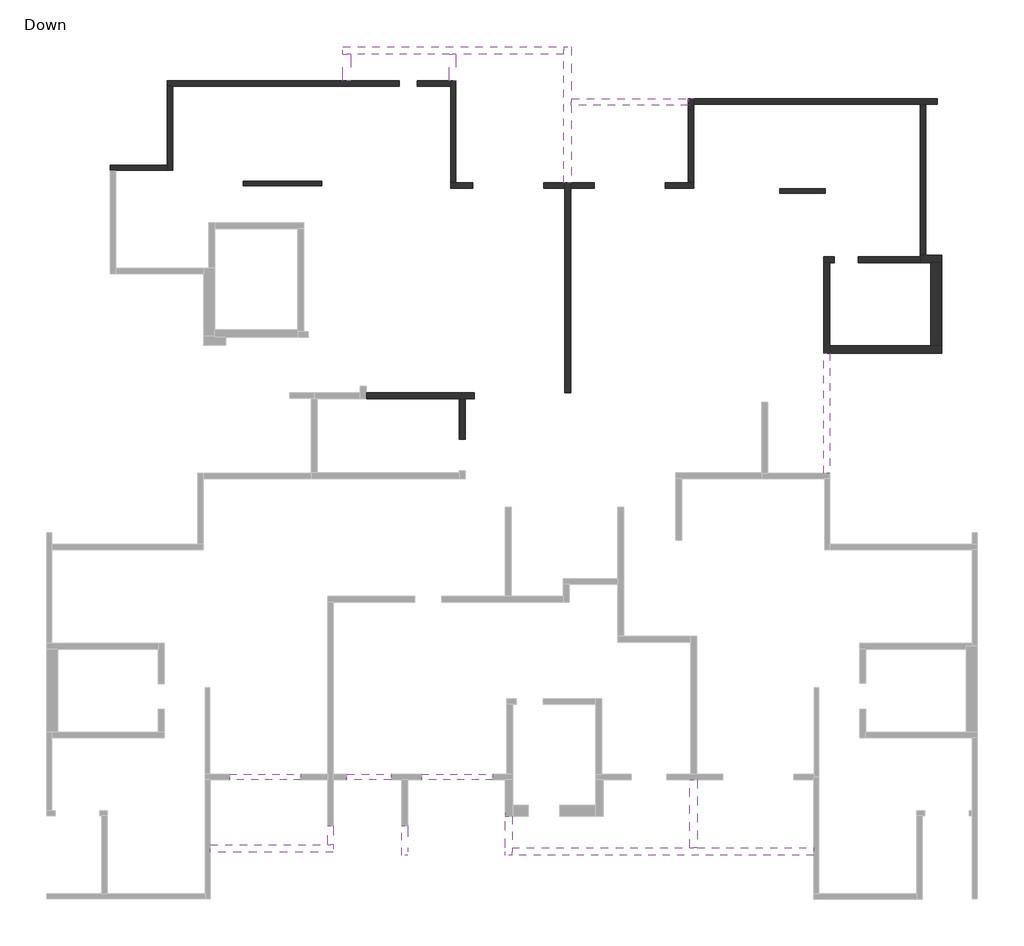
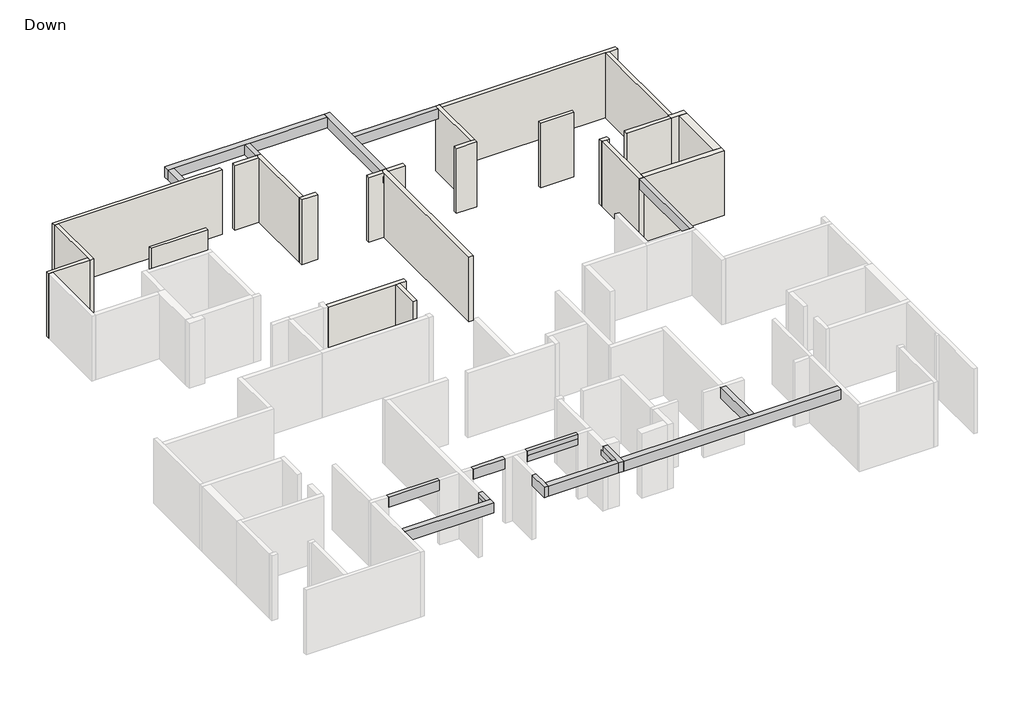
# One storey, part 3 of 3: 23 walls, 15 beams.
"""IFC4 building model written with IfcOpenShell, lengths in millimetres."""

from ifc_helpers import new_model, si_unit, frame, origin, place, context, project, spatial, polyline, outline, extrude, faceted_brep, element, save

model = new_model("IFC4")

# Units and contexts
model_context = context("Model", 3, world=origin())
ifc_project = project(units=[si_unit("LENGTHUNIT", "METRE", prefix="MILLI")], contexts=[model_context])

# Site, building, storey
site = spatial("IfcSite", under=ifc_project)
building = spatial("IfcBuilding", under=site)
storey = spatial("IfcBuildingStorey", under=building, Name="Down", Elevation=0.0)

# Beams
placement = place(None, origin())
element("IfcBeam", 1, ObjectType="Concrete Rectengular Beam : 18/50", at=placement, inside=storey, context=model_context, shape_type="Brep", body=[
    faceted_brep([(-10116.2830918, -11344.051338, 3200.0), (-10116.2830918, -11524.051338, 3200.0), (-10116.2830918, -11524.051338, 2700.0), (-10116.2830918, -11344.051338, 2700.0), (-10116.2830918, -11344.051338, 3000.0), (-12517.1627599, -11344.051338, 2700.0), (-12517.1627599, -11524.051338, 2700.0), (-12517.1627599, -11524.051338, 3200.0), (-12517.1627599, -11344.051338, 3200.0), (-12517.1627599, -11344.051338, 3000.0)], [[[0, 1, 2, 3, 4]], [[5, 6, 7, 8, 9]], [[1, 0, 8, 7]], [[2, 1, 7, 6]], [[3, 2, 6, 5]], [[8, 0, 4, 3, 5, 9]]]),
])
element("IfcBeam", 2, ObjectType="Concrete Rectengular Beam : 18/50", at=placement, inside=storey, context=model_context, shape_type="Brep", body=[
    faceted_brep([(-7066.175208, -11524.051338, 3200.0), (-7066.175208, -11344.051338, 3200.0), (-8566.988486, -11344.051338, 3200.0), (-8566.988486, -11524.051338, 3200.0), (-7066.175208, -11524.051338, 2700.0), (-8566.988486, -11524.051338, 2700.0), (-7066.175208, -11344.051338, 2700.0), (-8566.988486, -11344.051338, 2700.0), (-7066.175208, -11344.051338, 3000.0), (-8566.988486, -11344.051338, 3000.0)], [[[0, 1, 2, 3]], [[4, 0, 3, 5]], [[6, 4, 5, 7]], [[2, 1, 8, 6, 7, 9]], [[1, 0, 4, 6, 8]], [[3, 2, 9, 7, 5]]]),
])
element("IfcBeam", 3, ObjectType="Concrete Rectengular Beam : 18/50", at=placement, inside=storey, context=model_context, shape_type="Brep", body=[
    faceted_brep([(-3636.648237, -11344.051338, 3200.0), (-6035.4200213, -11344.051338, 3200.0), (-6035.4200213, -11519.051338, 3200.0), (-3636.648237, -11519.051338, 3200.0), (-6035.4200213, -11524.051338, 2700.0), (-3636.648237, -11524.051338, 2700.0), (-3636.648237, -11524.051338, 2980.0), (-6035.4200213, -11524.051338, 2980.0), (-3636.648237, -11344.051338, 2700.0), (-6035.4200213, -11344.051338, 2700.0), (-6035.4200213, -11344.051338, 3000.0), (-3636.648237, -11344.051338, 3000.0), (-3636.648237, -11519.051338, 2980.0), (-6035.4200213, -11519.051338, 2980.0)], [[[0, 1, 2, 3]], [[4, 5, 6, 7]], [[8, 5, 4, 9]], [[9, 10, 1, 0, 11, 8]], [[5, 8, 11, 0, 3, 12, 6]], [[9, 4, 7, 13, 2, 1, 10]], [[12, 13, 7, 6]], [[13, 12, 3, 2]]]),
])
element("IfcBeam", 4, ObjectType="Concrete Rectengular Beam : 20/50", at=placement, inside=storey, context=model_context, shape_type="SweptSolid", body=[
    extrude(outline(polyline([(2700.0, -9216.2167018), (2700.0, -9016.2167018), (3200.0, -9016.2167018), (3200.0, -9211.2167018), (2980.0, -9211.2167018), (2980.0, -9216.2167018), (2700.0, -9216.2167018)])), frame((0.0, -13713.3127488, 0.0), z_axis=(0.0, 1.0, 0.0), x_axis=(0.0, 0.0, 1.0)), (0.0, 0.0, 1.0), 645.0124481),
])
element("IfcBeam", 5, ObjectType="Concrete Rectengular Beam : 20/50", at=placement, inside=storey, context=model_context, shape_type="Brep", body=[
    faceted_brep([(-6516.0175316, -13068.3003006, 3200.0), (-6516.0175316, -13068.3003006, 2700.0), (-6716.0175316, -13068.3003006, 2700.0), (-6716.0175316, -13068.3003006, 3200.0), (-6716.0175316, -14074.491172, 3200.0), (-6516.0175316, -14074.491172, 3200.0), (-6516.0175316, -13814.491172, 3200.0), (-6716.0175316, -14074.491172, 2700.0), (-6516.0175316, -13814.491172, 2700.0), (-6516.0175316, -14074.491172, 2700.0)], [[[0, 1, 2, 3]], [[0, 3, 4, 5, 6]], [[3, 2, 7, 4]], [[2, 1, 8, 9, 7]], [[1, 0, 6, 5, 9, 8]], [[5, 4, 7, 9]]]),
])
element("IfcBeam", 6, ObjectType="Concrete Rectengular Beam : 20/50", at=placement, inside=storey, context=model_context, shape_type="Brep", body=[
    faceted_brep([(7535.1359953, -1184.051338, 3200.0), (7735.1359953, -1184.051338, 3200.0), (7735.1359953, 2875.7328944, 3200.0), (7535.1359953, 2875.7328944, 3200.0), (7535.1359953, -1184.051338, 2700.0), (7535.1359953, -1184.051338, 3000.0), (7535.1359953, 2875.7328944, 2700.0), (7735.1359953, -1184.051338, 2700.0), (7735.1359953, 2875.7328944, 2700.0)], [[[0, 1, 2, 3]], [[4, 5, 0, 3, 6]], [[7, 4, 6, 8]], [[1, 7, 8, 2]], [[1, 0, 5, 4, 7]], [[3, 2, 8, 6]]]),
])
element("IfcBeam", 7, ObjectType="Concrete Rectengular Beam : 22/50", at=placement, inside=storey, context=model_context, shape_type="Brep", body=[
    faceted_brep([(3133.8745845, 11456.9279151, 3200.0), (3133.8745845, 11457.7079981, 3200.0), (-986.7976146, 11457.7079981, 3200.0), (-986.7976146, 11237.7079981, 3200.0), (2953.8745845, 11237.7079981, 3200.0), (2953.8745845, 11456.9279151, 3200.0), (3133.8745845, 11457.7079981, 2700.0), (-986.7976146, 11457.7079981, 2700.0), (3133.8745845, 11456.9279151, 2700.0), (2953.8745845, 11456.9279151, 2700.0), (2953.8745845, 11237.7079981, 2700.0), (-986.7976146, 11237.7079981, 2700.0), (2953.8745845, 11237.7079981, 2980.0), (-986.7976146, 11237.7079981, 2980.0)], [[[0, 1, 2, 3, 4, 5]], [[1, 6, 7, 2]], [[6, 8, 9, 10, 11, 7]], [[10, 12, 4, 3, 13, 11]], [[6, 1, 0, 8]], [[9, 5, 4, 12, 10]], [[5, 9, 8, 0]], [[3, 2, 7, 11, 13]]]),
])
element("IfcBeam", 8, ObjectType="Concrete Rectengular Beam : 23/50", at=placement, inside=storey, context=model_context, shape_type="Brep", body=[
    faceted_brep([(-3216.3411831, -12636.8603469, 2700.0), (-3220.4458666, -12636.8603469, 2700.0), (-3220.4458666, -12636.8603469, 2980.0), (-3216.3411831, -12636.8603469, 2980.0), (-3220.4458666, -14074.491172, 3200.0), (-2990.4458666, -14074.491172, 3200.0), (-2990.4458666, -13814.491172, 3200.0), (-2990.4458666, -12754.2256118, 3200.0), (-3211.3411831, -12754.2256118, 3200.0), (-3211.3411831, -13814.491172, 3200.0), (-3220.4458666, -13814.491172, 3200.0), (-3220.4458666, -13814.491172, 2700.0), (-3220.4458666, -14074.491172, 2700.0), (-3220.4458666, -13814.491172, 2980.0), (-3216.3411831, -12754.2256118, 2700.0), (-2990.4458666, -12754.2256118, 2700.0), (-2990.4458666, -13814.491172, 2700.0), (-2990.4458666, -14074.491172, 2700.0), (-3216.3411831, -12754.2256118, 2980.0), (-3211.3411831, -12754.2256118, 2980.0), (-3211.3411831, -13814.491172, 2980.0)], [[[0, 1, 2, 3]], [[4, 5, 6, 7, 8, 9, 10]], [[1, 11, 12, 4, 10, 13, 2]], [[1, 0, 14, 15, 16, 17, 12, 11]], [[15, 7, 6, 5, 17, 16]], [[14, 0, 3, 18]], [[15, 14, 18, 19, 8, 7]], [[5, 4, 12, 17]], [[20, 19, 18, 3, 2, 13]], [[20, 9, 8, 19]], [[9, 20, 13, 10]]]),
])
element("IfcBeam", 9, ObjectType="Concrete Rectengular Beam : 23/50", at=placement, inside=storey, context=model_context, shape_type="Brep", body=[
    faceted_brep([(-5116.3826769, 12066.1063384, 3200.0), (-5065.7934653, 12066.1063384, 3200.0), (-4886.3826769, 12066.1063384, 3200.0), (-4886.3826769, 12957.7411932, 3200.0), (-5116.3826769, 12957.7411932, 3200.0), (-4886.3826769, 12957.7411932, 2700.0), (-4886.3826769, 12957.7411932, 2980.0), (-4886.3826769, 12066.1063384, 2980.0), (-4886.3826769, 12066.1063384, 2700.0), (-5116.3826769, 12066.1063384, 2700.0), (-5116.3826769, 12957.7411932, 2700.0), (-5116.3826769, 12066.1063384, 2980.0), (-5116.3826769, 12957.7411932, 2980.0)], [[[0, 1, 2, 3, 4]], [[5, 6, 3, 2, 7, 8]], [[8, 9, 10, 5]], [[9, 11, 0, 4, 12, 10]], [[0, 11, 9, 8, 7, 2, 1]], [[4, 3, 6, 5, 10, 12]]]),
])
element("IfcBeam", 10, ObjectType="Concrete Rectengular Beam : 26/50", at=placement, inside=storey, context=model_context, shape_type="Brep", body=[
    faceted_brep([(-13167.6689839, -13713.3127488, 3200.0), (-13167.6689839, -13973.3127488, 3200.0), (-9016.2167018, -13973.3127488, 3200.0), (-9016.2167018, -13713.3127488, 3200.0), (-9211.2167018, -13713.3127488, 3200.0), (-13167.6689839, -13973.3127488, 2700.0), (-9016.2167018, -13973.3127488, 2700.0), (-13167.6689839, -13713.3127488, 2700.0), (-9216.2167018, -13713.3127488, 2700.0), (-9016.2167018, -13713.3127488, 2700.0), (-13167.6689839, -13713.3127488, 2980.0)], [[[0, 1, 2, 3, 4]], [[1, 5, 6, 2]], [[5, 7, 8, 9, 6]], [[7, 10, 0, 4, 3, 9, 8]], [[1, 0, 10, 7, 5]], [[3, 2, 6, 9]]]),
])
element("IfcBeam", 11, ObjectType="Concrete Rectengular Beam : 26/50", at=placement, inside=storey, context=model_context, shape_type="Brep", body=[
    faceted_brep([(7185.3434642, -14074.491172, 3200.0), (7185.3434642, -13814.491172, 3200.0), (3265.0530078, -13814.491172, 3200.0), (3005.0530078, -13814.491172, 3200.0), (-2990.4458666, -13814.491172, 3200.0), (-2990.4458666, -14074.491172, 3200.0), (7185.3434642, -14074.491172, 2700.0), (-2990.4458666, -14074.491172, 2700.0), (7185.3434642, -13814.491172, 2700.0), (-2990.4458666, -13814.491172, 2700.0), (3005.0530078, -13814.491172, 2700.0), (3265.0530078, -13814.491172, 2700.0), (7185.3434642, -13814.491172, 2980.0)], [[[0, 1, 2, 3, 4, 5]], [[6, 0, 5, 7]], [[8, 6, 7, 9, 10, 11]], [[1, 12, 8, 11, 10, 9, 4, 3, 2]], [[1, 0, 6, 8, 12]], [[5, 4, 9, 7]]]),
    faceted_brep([(-6516.0175316, -14074.491172, 3200.0), (-6516.0175316, -13814.491172, 3200.0), (-6516.0175316, -13814.491172, 2980.0), (-6516.0175316, -13814.491172, 2700.0), (-6516.0175316, -14074.491172, 2700.0), (-3220.4458666, -13814.491172, 3200.0), (-3220.4458666, -14074.491172, 3200.0), (-3220.4458666, -14074.491172, 2700.0), (-3220.4458666, -13814.491172, 2700.0), (-3220.4458666, -13814.491172, 2980.0)], [[[0, 1, 2, 3, 4]], [[5, 6, 7, 8, 9]], [[1, 0, 6, 5]], [[0, 4, 7, 6]], [[4, 3, 8, 7]], [[3, 2, 1, 5, 9, 8]]]),
])
element("IfcBeam", 12, ObjectType="Concrete Rectengular Beam : 26/50", at=placement, inside=storey, context=model_context, shape_type="Brep", body=[
    faceted_brep([(3265.0530078, -11524.051338, 3200.0), (3005.0530078, -11524.051338, 3200.0), (3005.0530078, -13814.491172, 3200.0), (3265.0530078, -13814.491172, 3200.0), (3005.0530078, -11524.051338, 2700.0), (3005.0530078, -13814.491172, 2700.0), (3265.0530078, -11524.051338, 2700.0), (3265.0530078, -13814.491172, 2700.0), (3265.0530078, -11524.051338, 2980.0), (3265.0530078, -13814.491172, 2980.0)], [[[0, 1, 2, 3]], [[1, 4, 5, 2]], [[4, 6, 7, 5]], [[6, 8, 0, 3, 9, 7]], [[1, 0, 8, 6, 4]], [[3, 2, 5, 7, 9]]]),
])
element("IfcBeam", 13, ObjectType="Concrete Rectengular Beam : 26/50", at=placement, inside=storey, context=model_context, shape_type="Brep", body=[
    faceted_brep([(-1246.7976146, 8617.6084131, 3200.0), (-1216.7976146, 8617.6084131, 3200.0), (-1016.7976146, 8617.6084131, 3200.0), (-986.7976146, 8617.6084131, 3200.0), (-986.7976146, 11237.7079981, 3200.0), (-986.7976146, 11457.7079981, 3200.0), (-986.7976146, 13217.7411932, 3200.0), (-1246.7976146, 13217.7411932, 3200.0), (-1246.7976146, 12957.7411932, 3200.0), (-986.7976146, 8617.6084131, 2980.0), (-986.7976146, 8617.6084131, 2700.0), (-986.7976146, 11237.7079981, 2700.0), (-986.7976146, 11457.7079981, 2700.0), (-986.7976146, 13217.7411932, 2700.0), (-1246.7976146, 8617.6084131, 2700.0), (-1246.7976146, 12957.7411932, 2700.0), (-1246.7976146, 13217.7411932, 2700.0), (-1246.7976146, 8617.6084131, 2980.0)], [[[0, 1, 2, 3, 4, 5, 6, 7, 8]], [[3, 9, 10, 11, 12, 13, 6, 5, 4]], [[10, 14, 15, 16, 13, 12, 11]], [[0, 17, 14, 10, 9, 3, 2, 1]], [[14, 17, 0, 8, 7, 16, 15]], [[7, 6, 13, 16]]]),
    faceted_brep([(-1246.7976146, 8435.2155047, 2700.0), (-1246.7976146, 8435.2155047, 3000.0), (-1246.7976146, 8437.6084131, 3000.0), (-1246.7976146, 8437.6084131, 2700.0), (-1216.7976146, 8435.2155047, 2700.0), (-1216.7976146, 8435.2155047, 3000.0), (-1216.7976146, 8437.6084131, 2700.0), (-1216.7976146, 8437.6084131, 3000.0)], [[[0, 1, 2, 3]], [[1, 0, 4, 5]], [[6, 3, 2, 7]], [[1, 5, 7, 2]], [[4, 6, 7, 5]], [[3, 6, 4, 0]]]),
])
element("IfcBeam", 14, ObjectType="Concrete Rectengular Beam : 26/50", at=placement, inside=storey, context=model_context, shape_type="Brep", body=[
    faceted_brep([(-8695.5693989, 13217.7411932, 3200.0), (-8695.5693989, 12957.7411932, 3200.0), (-8435.5693989, 12957.7411932, 3200.0), (-5116.3826769, 12957.7411932, 3200.0), (-4886.3826769, 12957.7411932, 3200.0), (-1246.7976146, 12957.7411932, 3200.0), (-1246.7976146, 13217.7411932, 3200.0), (-8695.5693989, 13217.7411932, 2700.0), (-1246.7976146, 13217.7411932, 2700.0), (-8695.5693989, 12957.7411932, 2700.0), (-1246.7976146, 12957.7411932, 2700.0), (-4886.3826769, 12957.7411932, 2700.0), (-5116.3826769, 12957.7411932, 2700.0), (-8435.5693989, 12957.7411932, 2700.0), (-1246.7976146, 12957.7411932, 2980.0)], [[[0, 1, 2, 3, 4, 5, 6]], [[7, 0, 6, 8]], [[9, 7, 8, 10, 11, 12, 13]], [[1, 9, 13, 12, 11, 10, 14, 5, 4, 3, 2]], [[6, 5, 14, 10, 8]], [[1, 0, 7, 9]]]),
])
element("IfcBeam", 15, ObjectType="Concrete Rectengular Beam : 26/50", at=placement, inside=storey, context=model_context, shape_type="Brep", body=[
    faceted_brep([(-8695.5693989, 12066.1063384, 3200.0), (-8435.5693989, 12066.1063384, 3200.0), (-8435.5693989, 12957.7411932, 3200.0), (-8695.5693989, 12957.7411932, 3200.0), (-8695.5693989, 12066.1063384, 2700.0), (-8695.5693989, 12957.7411932, 2700.0), (-8435.5693989, 12066.1063384, 2700.0), (-8435.5693989, 12957.7411932, 2700.0), (-8435.5693989, 12066.1063384, 2980.0), (-8435.5693989, 12957.7411932, 2980.0)], [[[0, 1, 2, 3]], [[4, 0, 3, 5]], [[6, 4, 5, 7]], [[1, 8, 6, 7, 9, 2]], [[1, 0, 4, 6, 8]], [[3, 2, 9, 7, 5]]]),
])

# Walls
element("IfcWall", 16, ObjectType="15", at=placement, inside=storey, context=model_context, shape_type="Brep", body=[
    faceted_brep([(-12061.8598553, 8516.4299898, 0.0), (-9416.4656644, 8516.4299898, 0.0), (-9416.4656644, 8516.4299898, 3000.0), (-9416.4656644, 8516.4299898, 3200.0), (-12061.8598553, 8516.4299898, 3200.0), (-12061.8598553, 8516.4299898, 3000.0), (-12061.8598553, 8666.4299898, 0.0), (-12061.8598553, 8666.4299898, 3000.0), (-12061.8598553, 8666.4299898, 3200.0), (-9416.4656644, 8666.4299898, 3200.0), (-9416.4656644, 8666.4299898, 3000.0), (-9416.4656644, 8666.4299898, 0.0)], [[[0, 1, 2, 3, 4, 5]], [[6, 7, 8, 9, 10, 11]], [[1, 0, 6, 11]], [[3, 2, 1, 11, 10, 9]], [[4, 3, 9, 8]], [[0, 5, 4, 8, 7, 6]]]),
])
element("IfcWall", 17, ObjectType="15", at=placement, inside=storey, context=model_context, shape_type="Brep", body=[
    faceted_brep([(6036.4306011, 8275.7909857, 0.0), (7585.7252069, 8275.7909857, 0.0), (7585.7252069, 8275.7909857, 3000.0), (7585.7252069, 8275.7909857, 3200.0), (6036.4306011, 8275.7909857, 3200.0), (6036.4306011, 8275.7909857, 3000.0), (6036.4306011, 8425.7909857, 0.0), (6036.4306011, 8425.7909857, 3000.0), (6036.4306011, 8425.7909857, 3200.0), (7585.7252069, 8425.7909857, 3200.0), (7585.7252069, 8425.7909857, 3000.0), (7585.7252069, 8425.7909857, 0.0)], [[[0, 1, 2, 3, 4, 5]], [[6, 7, 8, 9, 10, 11]], [[1, 0, 6, 11]], [[3, 2, 1, 11, 10, 9]], [[4, 3, 9, 8]], [[0, 5, 4, 8, 7, 6]]]),
])
element("IfcWall", 18, ObjectType="18", at=placement, inside=storey, context=model_context, shape_type="Brep", body=[
    faceted_brep([(-1216.7976146, 8617.6084131, 0.0), (-1916.615042, 8617.6084131, 0.0), (-1916.615042, 8617.6084131, 3000.0), (-1916.615042, 8617.6084131, 3200.0), (-1246.7976146, 8617.6084131, 3200.0), (-1216.7976146, 8617.6084131, 3200.0), (-1216.7976146, 8437.6084131, 0.0), (-1216.7976146, 8437.6084131, 3000.0), (-1216.7976146, 8437.6084131, 3200.0), (-1916.615042, 8437.6084131, 3200.0), (-1916.615042, 8437.6084131, 3000.0), (-1916.615042, 8437.6084131, 0.0)], [[[0, 1, 2, 3, 4, 5]], [[6, 7, 8, 9, 10, 11]], [[1, 0, 6, 11]], [[3, 2, 1, 11, 10, 9]], [[5, 4, 3, 9, 8]], [[0, 5, 8, 7, 6]]]),
])
element("IfcWall", 19, ObjectType="18", at=placement, inside=storey, context=model_context, shape_type="Brep", body=[
    faceted_brep([(-1016.7976146, 8437.6084131, 0.0), (-215.5528014, 8437.6084131, 0.0), (-215.5528014, 8437.6084131, 3000.0), (-215.5528014, 8437.6084131, 3200.0), (-1016.7976146, 8437.6084131, 3200.0), (-1016.7976146, 8437.6084131, 3000.0), (-1016.7976146, 8617.6084131, 0.0), (-1016.7976146, 8617.6084131, 3200.0), (-986.7976146, 8617.6084131, 3200.0), (-215.5528014, 8617.6084131, 3200.0), (-215.5528014, 8617.6084131, 3000.0), (-215.5528014, 8617.6084131, 0.0)], [[[0, 1, 2, 3, 4, 5]], [[6, 7, 8, 9, 10, 11]], [[1, 0, 6, 11]], [[3, 2, 1, 11, 10, 9]], [[4, 3, 9, 8, 7]], [[0, 5, 4, 7, 6]]]),
])
element("IfcWall", 20, ObjectType="18", at=placement, inside=storey, context=model_context, shape_type="Brep", body=[
    faceted_brep([(-4315.3868263, 8617.6084131, 0.0), (-4885.7934653, 8617.6084131, 0.0), (-5065.7934653, 8617.6084131, 0.0), (-5065.7934653, 8617.6084131, 3200.0), (-4885.7934653, 8617.6084131, 3200.0), (-4315.3868263, 8617.6084131, 3200.0), (-4315.3868263, 8617.6084131, 3000.0), (-4315.3868263, 8437.6084131, 0.0), (-4315.3868263, 8437.6084131, 3000.0), (-4315.3868263, 8437.6084131, 3200.0), (-5065.7934653, 8437.6084131, 3200.0), (-5065.7934653, 8437.6084131, 3000.0), (-5065.7934653, 8437.6084131, 0.0)], [[[0, 1, 2, 3, 4, 5, 6]], [[7, 8, 9, 10, 11, 12]], [[2, 1, 0, 7, 12]], [[5, 4, 3, 10, 9]], [[0, 6, 5, 9, 8, 7]], [[3, 2, 12, 11, 10]]]),
])
element("IfcWall", 21, ObjectType="18", at=placement, inside=storey, context=model_context, shape_type="Brep", body=[
    faceted_brep([(-4885.7934653, 8617.6084131, 0.0), (-4885.7934653, 12066.1063384, 0.0), (-4885.7934653, 12066.1063384, 2980.0), (-4885.7934653, 12066.1063384, 3200.0), (-4885.7934653, 8617.6084131, 3200.0), (-4885.7934653, 8617.6084131, 2980.0), (-5065.7934653, 8617.6084131, 0.0), (-5065.7934653, 8617.6084131, 3200.0), (-5065.7934653, 11886.1063384, 3200.0), (-5065.7934653, 12066.1063384, 3200.0), (-5065.7934653, 12066.1063384, 0.0), (-5065.7934653, 11886.1063384, 0.0), (-4886.3826769, 12066.1063384, 3200.0)], [[[0, 1, 2, 3, 4, 5]], [[6, 7, 8, 9, 10, 11]], [[1, 0, 6, 11, 10]], [[4, 3, 12, 9, 8, 7]], [[0, 5, 4, 7, 6]], [[3, 2, 1, 10, 9, 12]]]),
])
element("IfcWall", 22, ObjectType="18", at=placement, inside=storey, context=model_context, shape_type="Brep", body=[
    faceted_brep([(-5065.7934653, 12066.1063384, 0.0), (-6191.4034238, 12066.1063384, 0.0), (-6191.4034238, 12066.1063384, 2980.0), (-6191.4034238, 12066.1063384, 3200.0), (-5116.3826769, 12066.1063384, 3200.0), (-5065.7934653, 12066.1063384, 3200.0), (-5065.7934653, 11886.1063384, 0.0), (-5065.7934653, 11886.1063384, 3000.0), (-5065.7934653, 11886.1063384, 3200.0), (-6191.4034238, 11886.1063384, 3200.0), (-6191.4034238, 11886.1063384, 2980.0), (-6191.4034238, 11886.1063384, 0.0)], [[[0, 1, 2, 3, 4, 5]], [[6, 7, 8, 9, 10, 11]], [[1, 0, 6, 11]], [[3, 2, 1, 11, 10, 9]], [[5, 4, 3, 9, 8]], [[0, 5, 8, 7, 6]]]),
])
element("IfcWall", 23, ObjectType="18", at=placement, inside=storey, context=model_context, shape_type="Brep", body=[
    faceted_brep([(-6790.0424279, 12066.1063384, 0.0), (-14627.1544611, 12066.1063384, 0.0), (-14627.1544611, 12066.1063384, 3200.0), (-8435.5693989, 12066.1063384, 3200.0), (-6790.0424279, 12066.1063384, 3200.0), (-6790.0424279, 12066.1063384, 2980.0), (-6790.0424279, 11886.1063384, 0.0), (-6790.0424279, 11886.1063384, 2980.0), (-6790.0424279, 11886.1063384, 3200.0), (-14447.1544611, 11886.1063384, 3200.0), (-14627.1544611, 11886.1063384, 3200.0), (-14627.1544611, 11886.1063384, 0.0), (-14447.1544611, 11886.1063384, 0.0)], [[[0, 1, 2, 3, 4, 5]], [[6, 7, 8, 9, 10, 11, 12]], [[1, 0, 6, 12, 11]], [[4, 3, 2, 10, 9, 8]], [[0, 5, 4, 8, 7, 6]], [[2, 1, 11, 10]]]),
])
element("IfcWall", 24, ObjectType="18", at=placement, inside=storey, context=model_context, shape_type="Brep", body=[
    faceted_brep([(-14627.1544611, 11886.1063384, 0.0), (-14627.1544611, 9217.0772927, 0.0), (-14627.1544611, 9037.0772927, 0.0), (-14627.1544611, 9037.0772927, 3200.0), (-14627.1544611, 9217.0772927, 3200.0), (-14627.1544611, 11886.1063384, 3200.0), (-14447.1544611, 11886.1063384, 0.0), (-14447.1544611, 11886.1063384, 3000.0), (-14447.1544611, 11886.1063384, 3200.0), (-14447.1544611, 9037.0772927, 3200.0), (-14447.1544611, 9037.0772927, 3000.0), (-14447.1544611, 9037.0772927, 0.0)], [[[0, 1, 2, 3, 4, 5]], [[6, 7, 8, 9, 10, 11]], [[2, 1, 0, 6, 11]], [[5, 4, 3, 9, 8]], [[0, 5, 8, 7, 6]], [[3, 2, 11, 10, 9]]]),
])
element("IfcWall", 25, ObjectType="18", at=placement, inside=storey, context=model_context, shape_type="Brep", body=[
    faceted_brep([(-14627.1544611, 9217.0772927, 0.0), (-16547.4366188, 9217.0772927, 0.0), (-16547.4366188, 9217.0772927, 3200.0), (-14627.1544611, 9217.0772927, 3200.0), (-14627.1544611, 9037.0772927, 0.0), (-14627.1544611, 9037.0772927, 3200.0), (-16367.4366188, 9037.0772927, 3200.0), (-16547.4366188, 9037.0772927, 3200.0), (-16547.4366188, 9037.0772927, 0.0), (-16367.4366188, 9037.0772927, 0.0)], [[[0, 1, 2, 3]], [[4, 5, 6, 7, 8, 9]], [[1, 0, 4, 9, 8]], [[3, 2, 7, 6, 5]], [[0, 3, 5, 4]], [[2, 1, 8, 7]]]),
])
element("IfcWall", 26, ObjectType="18", at=placement, inside=storey, context=model_context, shape_type="Brep", body=[
    faceted_brep([(2183.2189829, 8437.6084131, 0.0), (3133.8745845, 8437.6084131, 0.0), (3133.8745845, 8437.6084131, 3000.0), (3133.8745845, 8437.6084131, 3200.0), (2183.2189829, 8437.6084131, 3200.0), (2183.2189829, 8437.6084131, 3000.0), (2183.2189829, 8617.6084131, 0.0), (2183.2189829, 8617.6084131, 3000.0), (2183.2189829, 8617.6084131, 3200.0), (2953.8745845, 8617.6084131, 3200.0), (3133.8745845, 8617.6084131, 3200.0), (3133.8745845, 8617.6084131, 0.0), (2953.8745845, 8617.6084131, 0.0)], [[[0, 1, 2, 3, 4, 5]], [[6, 7, 8, 9, 10, 11, 12]], [[1, 0, 6, 12, 11]], [[4, 3, 10, 9, 8]], [[0, 5, 4, 8, 7, 6]], [[3, 2, 1, 11, 10]]]),
])
element("IfcWall", 27, ObjectType="18", at=placement, inside=storey, context=model_context, shape_type="Brep", body=[
    faceted_brep([(3133.8745845, 8617.6084131, 0.0), (3133.8745845, 11276.9279151, 0.0), (3133.8745845, 11456.9279151, 0.0), (3133.8745845, 11456.9279151, 3200.0), (3133.8745845, 11276.9279151, 3200.0), (3133.8745845, 8617.6084131, 3200.0), (2953.8745845, 8617.6084131, 0.0), (2953.8745845, 8617.6084131, 2980.0), (2953.8745845, 8617.6084131, 3200.0), (2953.8745845, 11237.7079981, 3200.0), (2953.8745845, 11456.9279151, 3200.0), (2953.8745845, 11456.9279151, 0.0)], [[[0, 1, 2, 3, 4, 5]], [[6, 7, 8, 9, 10, 11]], [[2, 1, 0, 6, 11]], [[5, 4, 3, 10, 9, 8]], [[0, 5, 8, 7, 6]], [[3, 2, 11, 10]]]),
])
element("IfcWall", 28, ObjectType="18", at=placement, inside=storey, context=model_context, shape_type="Brep", body=[
    faceted_brep([(3133.8745845, 11276.9279151, 0.0), (10784.6629663, 11276.9279151, 0.0), (10964.6629663, 11276.9279151, 0.0), (11365.1608916, 11276.9279151, 0.0), (11365.1608916, 11276.9279151, 3200.0), (10964.6629663, 11276.9279151, 3200.0), (10784.6629663, 11276.9279151, 3200.0), (3133.8745845, 11276.9279151, 3200.0), (3133.8745845, 11276.9279151, 3000.0), (3133.8745845, 11456.9279151, 0.0), (3133.8745845, 11456.9279151, 3200.0), (11365.1608916, 11456.9279151, 3200.0), (11365.1608916, 11456.9279151, 0.0)], [[[0, 1, 2, 3, 4, 5, 6, 7, 8]], [[9, 10, 11, 12]], [[3, 2, 1, 0, 9, 12]], [[4, 3, 12, 11]], [[7, 6, 5, 4, 11, 10]], [[0, 8, 7, 10, 9]]]),
])
element("IfcWall", 29, ObjectType="18", at=placement, inside=storey, context=model_context, shape_type="Brep", body=[
    faceted_brep([(10784.6629663, 11276.9279151, 0.0), (10784.6629663, 6175.8407782, 0.0), (10784.6629663, 6175.8407782, 3200.0), (10784.6629663, 11276.9279151, 3200.0), (10784.6629663, 11276.9279151, 3000.0), (10964.6629663, 11276.9279151, 0.0), (10964.6629663, 11276.9279151, 3200.0), (10964.6629663, 6175.8407782, 3200.0), (10964.6629663, 6175.8407782, 0.0)], [[[0, 1, 2, 3, 4]], [[5, 6, 7, 8]], [[1, 0, 5, 8]], [[3, 2, 7, 6]], [[2, 1, 8, 7]], [[0, 4, 3, 6, 5]]]),
])
element("IfcWall", 30, ObjectType="20", at=placement, inside=storey, context=model_context, shape_type="Brep", body=[
    faceted_brep([(-1016.7976146, 1537.2266703, 0.0), (-1016.7976146, 8437.6084131, 0.0), (-1016.7976146, 8617.6084131, 0.0), (-1016.7976146, 8617.6084131, 3200.0), (-1016.7976146, 8437.6084131, 3200.0), (-1016.7976146, 1537.2266703, 3200.0), (-1016.7976146, 1537.2266703, 3000.0), (-1216.7976146, 1537.2266703, 0.0), (-1216.7976146, 1537.2266703, 3000.0), (-1216.7976146, 1537.2266703, 3200.0), (-1216.7976146, 8437.6084131, 3200.0), (-1216.7976146, 8617.6084131, 3200.0), (-1216.7976146, 8617.6084131, 0.0), (-1216.7976146, 8437.6084131, 0.0), (-1116.7976146, 1537.2266703, 3200.0)], [[[0, 1, 2, 3, 4, 5, 6]], [[7, 8, 9, 10, 11, 12, 13]], [[2, 1, 0, 7, 13, 12]], [[5, 4, 3, 11, 10, 9, 14]], [[0, 6, 5, 14, 9, 8, 7]], [[3, 2, 12, 11]]]),
])
element("IfcWall", 31, ObjectType="20", at=placement, inside=storey, context=model_context, shape_type="Brep", body=[
    faceted_brep([(10784.6629663, 6125.8407782, 0.0), (8690.2563273, 6125.8407782, 0.0), (8690.2563273, 6125.8407782, 3000.0), (8690.2563273, 6125.8407782, 3200.0), (10784.6629663, 6125.8407782, 3200.0), (10784.6629663, 6125.8407782, 3000.0), (10784.6629663, 5925.8407782, 0.0), (10784.6629663, 5925.8407782, 3200.0), (8690.2563273, 5925.8407782, 3200.0), (8690.2563273, 5925.8407782, 3000.0), (8690.2563273, 5925.8407782, 0.0), (8690.2563273, 5930.8407782, 3200.0)], [[[0, 1, 2, 3, 4, 5]], [[6, 7, 8, 9, 10]], [[1, 0, 6, 10]], [[3, 2, 1, 10, 9, 8, 11]], [[4, 3, 11, 8, 7]], [[0, 5, 4, 7, 6]]]),
])
element("IfcWall", 32, ObjectType="20", at=placement, inside=storey, context=model_context, shape_type="Brep", body=[
    faceted_brep([(7878.7210576, 6125.8407782, 0.0), (7535.1359953, 6125.8407782, 0.0), (7535.1359953, 6125.8407782, 3000.0), (7535.1359953, 6125.8407782, 3200.0), (7878.7210576, 6125.8407782, 3200.0), (7878.7210576, 6125.8407782, 3000.0), (7878.7210576, 5925.8407782, 0.0), (7878.7210576, 5925.8407782, 3000.0), (7878.7210576, 5925.8407782, 3200.0), (7735.1359953, 5925.8407782, 3200.0), (7535.1359953, 5925.8407782, 3200.0), (7535.1359953, 5925.8407782, 0.0), (7735.1359953, 5925.8407782, 0.0), (7878.7210576, 5930.8407782, 3200.0)], [[[0, 1, 2, 3, 4, 5]], [[6, 7, 8, 9, 10, 11, 12]], [[1, 0, 6, 12, 11]], [[4, 3, 10, 9, 8, 13]], [[0, 5, 4, 13, 8, 7, 6]], [[3, 2, 1, 11, 10]]]),
])
element("IfcWall", 33, ObjectType="20", at=placement, inside=storey, context=model_context, shape_type="Brep", body=[
    faceted_brep([(7535.1359953, 5925.8407782, 0.0), (7535.1359953, 2875.7328944, 0.0), (7535.1359953, 2875.7328944, 2700.0), (7535.1359953, 2875.7328944, 3200.0), (7535.1359953, 5925.8407782, 3200.0), (7735.1359953, 5925.8407782, 0.0), (7735.1359953, 5925.8407782, 3000.0), (7735.1359953, 5925.8407782, 3200.0), (7735.1359953, 3125.7328944, 3200.0), (7735.1359953, 2875.7328944, 3200.0), (7735.1359953, 2875.7328944, 2700.0), (7735.1359953, 2875.7328944, 0.0), (7735.1359953, 3125.7328944, 0.0)], [[[0, 1, 2, 3, 4]], [[5, 6, 7, 8, 9, 10, 11, 12]], [[1, 0, 5, 12, 11]], [[4, 3, 9, 8, 7]], [[0, 4, 7, 6, 5]], [[3, 2, 1, 11, 10, 9]]]),
])
element("IfcWall", 34, ObjectType="20", at=placement, inside=storey, context=model_context, shape_type="Brep", body=[
    faceted_brep([(-4566.2250005, -39.4704251, 0.0), (-4566.2250005, 1337.2266703, 0.0), (-4566.2250005, 1337.2266703, 3000.0), (-4566.2250005, 1337.2266703, 3200.0), (-4566.2250005, -39.4704251, 3200.0), (-4766.2250005, -39.4704251, 0.0), (-4766.2250005, -39.4704251, 3200.0), (-4766.2250005, 1337.2266703, 3200.0), (-4766.2250005, 1337.2266703, 0.0)], [[[0, 1, 2, 3, 4]], [[5, 6, 7, 8]], [[1, 0, 5, 8]], [[4, 3, 7, 6]], [[0, 4, 6, 5]], [[3, 2, 1, 8, 7]]]),
])
element("IfcWall", 35, ObjectType="20", at=placement, inside=storey, context=model_context, shape_type="Brep", body=[
    faceted_brep([(-4266.9054985, 1537.2266703, 0.0), (-7916.2250005, 1537.2266703, 0.0), (-7916.2250005, 1537.2266703, 3000.0), (-7916.2250005, 1537.2266703, 3200.0), (-4266.9054985, 1537.2266703, 3200.0), (-4266.9054985, 1537.2266703, 3000.0), (-4266.9054985, 1337.2266703, 0.0), (-4266.9054985, 1337.2266703, 3000.0), (-4266.9054985, 1337.2266703, 3200.0), (-4566.2250005, 1337.2266703, 3200.0), (-4766.2250005, 1337.2266703, 3200.0), (-7916.2250005, 1337.2266703, 3200.0), (-7916.2250005, 1337.2266703, 0.0), (-4766.2250005, 1337.2266703, 0.0), (-4566.2250005, 1337.2266703, 0.0)], [[[0, 1, 2, 3, 4, 5]], [[6, 7, 8, 9, 10, 11, 12, 13, 14]], [[1, 0, 6, 14, 13, 12]], [[4, 3, 11, 10, 9, 8]], [[0, 5, 4, 8, 7, 6]], [[3, 2, 1, 12, 11]]]),
])
element("IfcWall", 36, ObjectType="25", at=placement, inside=storey, context=model_context, shape_type="Brep", body=[
    faceted_brep([(7735.1359953, 2875.7328944, 0.0), (11504.2812235, 2875.7328944, 0.0), (11504.2812235, 2875.7328944, 3200.0), (7735.1359953, 2875.7328944, 3200.0), (7735.1359953, 3125.7328944, 0.0), (7735.1359953, 3125.7328944, 3000.0), (7735.1359953, 3125.7328944, 3200.0), (11134.2812235, 3125.7328944, 3200.0), (11504.2812235, 3125.7328944, 3200.0), (11504.2812235, 3125.7328944, 0.0), (11134.2812235, 3125.7328944, 0.0)], [[[0, 1, 2, 3]], [[4, 5, 6, 7, 8, 9, 10]], [[1, 0, 4, 10, 9]], [[3, 2, 8, 7, 6]], [[0, 3, 6, 5, 4]], [[2, 1, 9, 8]]]),
])
element("IfcWall", 37, ObjectType="25", at=placement, inside=storey, context=model_context, shape_type="Brep", body=[
    faceted_brep([(10784.6629663, 5925.8407782, 0.0), (11134.2812235, 5925.8407782, 0.0), (11504.2812235, 5925.8407782, 0.0), (11504.2812235, 5925.8407782, 3200.0), (11134.2812235, 5925.8407782, 3200.0), (10784.6629663, 5925.8407782, 3200.0), (10784.6629663, 6175.8407782, 0.0), (10784.6629663, 6175.8407782, 3200.0), (10964.6629663, 6175.8407782, 3200.0), (11504.2812235, 6175.8407782, 3200.0), (11504.2812235, 6175.8407782, 0.0), (10964.6629663, 6175.8407782, 0.0), (10784.6629663, 6125.8407782, 0.0), (10784.6629663, 6125.8407782, 3200.0)], [[[0, 1, 2, 3, 4, 5]], [[6, 7, 8, 9, 10, 11]], [[2, 1, 0, 12, 6, 11, 10]], [[5, 4, 3, 9, 8, 7, 13]], [[0, 5, 13, 7, 6, 12]], [[3, 2, 10, 9]]]),
])
element("IfcWall", 38, ObjectType="37", at=placement, inside=storey, context=model_context, shape_type="Brep", body=[
    faceted_brep([(11134.2812235, 5925.8407782, 0.0), (11134.2812235, 3125.7328944, 0.0), (11134.2812235, 3125.7328944, 3000.0), (11134.2812235, 3125.7328944, 3200.0), (11134.2812235, 5925.8407782, 3200.0), (11134.2812235, 5925.8407782, 3000.0), (11504.2812235, 5925.8407782, 0.0), (11504.2812235, 5925.8407782, 3200.0), (11504.2812235, 3125.7328944, 3200.0), (11504.2812235, 3125.7328944, 0.0)], [[[0, 1, 2, 3, 4, 5]], [[6, 7, 8, 9]], [[1, 0, 6, 9]], [[4, 3, 8, 7]], [[3, 2, 1, 9, 8]], [[0, 5, 4, 7, 6]]]),
])

save(model, "model.ifc")

# Revit data of these elements
# Type "Concrete Rectengular Beam : 18/50"
#   Length [instance default] = 152.4 cm
#   b = 18 cm
#   h = 50 cm
#   Structural Material [instance default] = Concrete
#   Assembly Code = ""
# Type "Concrete Rectengular Beam : 20/50"
#   Length [instance default] = 152.4 cm
#   b = 20 cm
#   h = 50 cm
#   Structural Material [instance default] = Concrete
#   Assembly Code = ""
# Type "Concrete Rectengular Beam : 22/50"
#   Length [instance default] = 152.4 cm
#   b = 22 cm
#   h = 50 cm
#   Structural Material [instance default] = Concrete
#   Assembly Code = ""
# Type "Concrete Rectengular Beam : 23/50"
#   Length [instance default] = 152.4 cm
#   b = 23 cm
#   h = 50 cm
#   Structural Material [instance default] = Concrete
#   Assembly Code = ""
# Type "Concrete Rectengular Beam : 26/50"
#   Length [instance default] = 152.4 cm
#   b = 26 cm
#   h = 50 cm
#   Structural Material [instance default] = Concrete
#   Assembly Code = ""
# Type "15"
#   Layers, outside or top first: 15 cm "Concrete" (function 1)
# Type "18"
#   Layers, outside or top first: 18 cm "Concrete" (function 1)
# Type "20"
#   Layers, outside or top first: 20 cm "Concrete" (function 1)
# Type "25"
#   Layers, outside or top first: 25 cm "Concrete" (function 1)
# Type "37"
#   Layers, outside or top first: 37 cm "Concrete" (function 1)
# Element 1 (IfcBeam, "Concrete Rectengular Beam : 18/50")
#   Comments = ""
#   Mark = "B1"
#   SOFiSTiK_AMG_Comments = ""
#   SOFiSTiK_AMG_Scheduled = yes
#   SOFiSTiK_AMG_Adjusted = yes
#   Structural Material = Concrete
#   Phase Created = New Construction
#   Materials on its faces: "Concrete"
# Element 2 (IfcBeam, "Concrete Rectengular Beam : 18/50")
#   Comments = ""
#   Mark = "B2"
#   SOFiSTiK_AMG_Comments = ""
#   SOFiSTiK_AMG_Scheduled = yes
#   SOFiSTiK_AMG_Adjusted = yes
#   Structural Material = Concrete
#   Phase Created = New Construction
#   Materials on its faces: "Concrete"
# Element 3 (IfcBeam, "Concrete Rectengular Beam : 18/50")
#   Comments = ""
#   Mark = "B3"
#   SOFiSTiK_AMG_Comments = ""
#   SOFiSTiK_AMG_Scheduled = yes
#   SOFiSTiK_AMG_Adjusted = yes
#   Structural Material = Concrete
#   Phase Created = New Construction
#   Materials on its faces: "Concrete"
# Element 4 (IfcBeam, "Concrete Rectengular Beam : 20/50")
#   Comments = ""
#   Mark = "B4"
#   SOFiSTiK_AMG_Comments = ""
#   SOFiSTiK_AMG_Scheduled = yes
#   SOFiSTiK_AMG_Adjusted = yes
#   Structural Material = Concrete
#   Phase Created = New Construction
#   Materials on its faces: "Concrete"
# Element 5 (IfcBeam, "Concrete Rectengular Beam : 20/50")
#   Comments = ""
#   Mark = "B5"
#   SOFiSTiK_AMG_Comments = ""
#   SOFiSTiK_AMG_Scheduled = yes
#   SOFiSTiK_AMG_Adjusted = yes
#   Structural Material = Concrete
#   Phase Created = New Construction
#   Materials on its faces: "Concrete"
# Element 6 (IfcBeam, "Concrete Rectengular Beam : 20/50")
#   Comments = ""
#   Mark = "B6"
#   SOFiSTiK_AMG_Comments = ""
#   SOFiSTiK_AMG_Scheduled = yes
#   SOFiSTiK_AMG_Adjusted = yes
#   Structural Material = Concrete
#   Phase Created = New Construction
#   Materials on its faces: "Concrete"
# Element 7 (IfcBeam, "Concrete Rectengular Beam : 22/50")
#   Comments = ""
#   Mark = "B7"
#   SOFiSTiK_AMG_Comments = ""
#   SOFiSTiK_AMG_Scheduled = yes
#   SOFiSTiK_AMG_Adjusted = yes
#   Structural Material = Concrete
#   Phase Created = New Construction
#   Materials on its faces: "Concrete"
# Element 8 (IfcBeam, "Concrete Rectengular Beam : 23/50")
#   Comments = ""
#   Mark = "B8"
#   SOFiSTiK_AMG_Comments = ""
#   SOFiSTiK_AMG_Scheduled = yes
#   SOFiSTiK_AMG_Adjusted = yes
#   Structural Material = Concrete
#   Phase Created = New Construction
#   Materials on its faces: "Concrete"
# Element 9 (IfcBeam, "Concrete Rectengular Beam : 23/50")
#   Comments = ""
#   Mark = "B9"
#   SOFiSTiK_AMG_Comments = ""
#   SOFiSTiK_AMG_Scheduled = yes
#   SOFiSTiK_AMG_Adjusted = yes
#   Structural Material = Concrete
#   Phase Created = New Construction
#   Materials on its faces: "Concrete"
# Element 10 (IfcBeam, "Concrete Rectengular Beam : 26/50")
#   Comments = ""
#   Mark = "B10"
#   SOFiSTiK_AMG_Comments = ""
#   SOFiSTiK_AMG_Scheduled = yes
#   SOFiSTiK_AMG_Adjusted = yes
#   Structural Material = Concrete
#   Phase Created = New Construction
#   Materials on its faces: "Concrete"
# Element 11 (IfcBeam, "Concrete Rectengular Beam : 26/50")
#   Comments = ""
#   Mark = "B11"
#   SOFiSTiK_AMG_Comments = ""
#   SOFiSTiK_AMG_Scheduled = yes
#   SOFiSTiK_AMG_Adjusted = yes
#   Structural Material = Concrete
#   Phase Created = New Construction
#   Materials on its faces: "Concrete"
# Element 12 (IfcBeam, "Concrete Rectengular Beam : 26/50")
#   Comments = ""
#   Mark = "B12"
#   SOFiSTiK_AMG_Comments = ""
#   SOFiSTiK_AMG_Scheduled = yes
#   SOFiSTiK_AMG_Adjusted = yes
#   Structural Material = Concrete
#   Phase Created = New Construction
#   Materials on its faces: "Concrete"
# Element 13 (IfcBeam, "Concrete Rectengular Beam : 26/50")
#   Comments = ""
#   Mark = "B13"
#   SOFiSTiK_AMG_Comments = ""
#   SOFiSTiK_AMG_Scheduled = yes
#   SOFiSTiK_AMG_Adjusted = yes
#   Structural Material = Concrete
#   Phase Created = New Construction
#   Materials on its faces: "Concrete"
# Element 14 (IfcBeam, "Concrete Rectengular Beam : 26/50")
#   Comments = ""
#   Mark = "B14"
#   SOFiSTiK_AMG_Comments = ""
#   SOFiSTiK_AMG_Scheduled = yes
#   SOFiSTiK_AMG_Adjusted = yes
#   Structural Material = Concrete
#   Phase Created = New Construction
#   Materials on its faces: "Concrete"
# Element 15 (IfcBeam, "Concrete Rectengular Beam : 26/50")
#   Comments = ""
#   Mark = "B15"
#   SOFiSTiK_AMG_Comments = ""
#   SOFiSTiK_AMG_Scheduled = yes
#   SOFiSTiK_AMG_Adjusted = yes
#   Structural Material = Concrete
#   Phase Created = New Construction
#   Materials on its faces: "Concrete"
# Element 16 (IfcWall, "15")
#   Comments = ""
#   Mark = "W97"
#   SOFiSTiK_EdgeZones = "W98"
#   SOFiSTiK_AMG_Comments = ""
#   Top Offset = 0 cm
#   Base Offset = 0 cm
#   wall height = 320 cm
#   SOFiSTiK_AMG_Scheduled = yes
#   SOFiSTiK_AMG_Adjusted = yes
#   Phase Created = New Construction
#   Base Constraint = Down
#   Top Constraint = Typical Floor
#   Materials on its faces: "Concrete"
# Element 17 (IfcWall, "15")
#   Comments = ""
#   Mark = "W98"
#   SOFiSTiK_EdgeZones = "W99"
#   SOFiSTiK_AMG_Comments = ""
#   Top Offset = 0 cm
#   Base Offset = 0 cm
#   wall height = 320 cm
#   SOFiSTiK_AMG_Scheduled = yes
#   SOFiSTiK_AMG_Adjusted = yes
#   Phase Created = New Construction
#   Base Constraint = Down
#   Top Constraint = Typical Floor
#   Materials on its faces: "Concrete"
# Element 18 (IfcWall, "18")
#   Comments = ""
#   Mark = "W40"
#   SOFiSTiK_EdgeZones = "W40"
#   SOFiSTiK_AMG_Comments = ""
#   Top Offset = 0 cm
#   Base Offset = 0 cm
#   wall height = 320 cm
#   SOFiSTiK_AMG_Scheduled = yes
#   SOFiSTiK_AMG_Adjusted = yes
#   Phase Created = New Construction
#   Base Constraint = Down
#   Top Constraint = Typical Floor
#   Materials on its faces: "Concrete"
# Element 19 (IfcWall, "18")
#   Comments = ""
#   Mark = "W41"
#   SOFiSTiK_EdgeZones = "W41"
#   SOFiSTiK_AMG_Comments = ""
#   Top Offset = 0 cm
#   Base Offset = 0 cm
#   wall height = 320 cm
#   SOFiSTiK_AMG_Scheduled = yes
#   SOFiSTiK_AMG_Adjusted = yes
#   Phase Created = New Construction
#   Base Constraint = Down
#   Top Constraint = Typical Floor
#   Materials on its faces: "Concrete"
# Element 20 (IfcWall, "18")
#   Comments = ""
#   Mark = "W42"
#   SOFiSTiK_EdgeZones = "W42"
#   SOFiSTiK_AMG_Comments = ""
#   Top Offset = 0 cm
#   Base Offset = 0 cm
#   wall height = 320 cm
#   SOFiSTiK_AMG_Scheduled = yes
#   SOFiSTiK_AMG_Adjusted = yes
#   Phase Created = New Construction
#   Base Constraint = Down
#   Top Constraint = Typical Floor
#   Materials on its faces: "Concrete"
# Element 21 (IfcWall, "18")
#   Comments = ""
#   Mark = "W43"
#   SOFiSTiK_EdgeZones = "W43"
#   SOFiSTiK_AMG_Comments = ""
#   Top Offset = 0 cm
#   Base Offset = 0 cm
#   wall height = 320 cm
#   SOFiSTiK_AMG_Scheduled = yes
#   SOFiSTiK_AMG_Adjusted = yes
#   Phase Created = New Construction
#   Base Constraint = Down
#   Top Constraint = Typical Floor
#   Materials on its faces: "Concrete"
# Element 22 (IfcWall, "18")
#   Comments = ""
#   Mark = "W44"
#   SOFiSTiK_EdgeZones = "W44"
#   SOFiSTiK_AMG_Comments = ""
#   Top Offset = 0 cm
#   Base Offset = 0 cm
#   wall height = 320 cm
#   SOFiSTiK_AMG_Scheduled = yes
#   SOFiSTiK_AMG_Adjusted = yes
#   Phase Created = New Construction
#   Base Constraint = Down
#   Top Constraint = Typical Floor
#   Materials on its faces: "Concrete"
# Element 23 (IfcWall, "18")
#   Comments = ""
#   Mark = "W45"
#   SOFiSTiK_EdgeZones = "W45"
#   SOFiSTiK_AMG_Comments = ""
#   Top Offset = 0 cm
#   Base Offset = 0 cm
#   wall height = 320 cm
#   SOFiSTiK_AMG_Scheduled = yes
#   SOFiSTiK_AMG_Adjusted = yes
#   Phase Created = New Construction
#   Base Constraint = Down
#   Top Constraint = Typical Floor
#   Materials on its faces: "Concrete"
# Element 24 (IfcWall, "18")
#   Comments = ""
#   Mark = "W46"
#   SOFiSTiK_EdgeZones = "W46"
#   SOFiSTiK_AMG_Comments = ""
#   Top Offset = 0 cm
#   Base Offset = 0 cm
#   wall height = 320 cm
#   SOFiSTiK_AMG_Scheduled = yes
#   SOFiSTiK_AMG_Adjusted = yes
#   Phase Created = New Construction
#   Base Constraint = Down
#   Top Constraint = Typical Floor
#   Materials on its faces: "Concrete"
# Element 25 (IfcWall, "18")
#   Comments = ""
#   Mark = "W47"
#   SOFiSTiK_EdgeZones = "W47"
#   SOFiSTiK_AMG_Comments = ""
#   Top Offset = 0 cm
#   Base Offset = 0 cm
#   wall height = 320 cm
#   SOFiSTiK_AMG_Scheduled = yes
#   SOFiSTiK_AMG_Adjusted = yes
#   Phase Created = New Construction
#   Base Constraint = Down
#   Top Constraint = Typical Floor
#   Materials on its faces: "Concrete"
# Element 26 (IfcWall, "18")
#   Comments = ""
#   Mark = "W51"
#   SOFiSTiK_EdgeZones = "W51"
#   SOFiSTiK_AMG_Comments = ""
#   Top Offset = 0 cm
#   Base Offset = 0 cm
#   wall height = 320 cm
#   SOFiSTiK_AMG_Scheduled = yes
#   SOFiSTiK_AMG_Adjusted = yes
#   Phase Created = New Construction
#   Base Constraint = Down
#   Top Constraint = Typical Floor
#   Materials on its faces: "Concrete"
# Element 27 (IfcWall, "18")
#   Comments = ""
#   Mark = "W52"
#   SOFiSTiK_EdgeZones = "W52"
#   SOFiSTiK_AMG_Comments = ""
#   Top Offset = 0 cm
#   Base Offset = 0 cm
#   wall height = 320 cm
#   SOFiSTiK_AMG_Scheduled = yes
#   SOFiSTiK_AMG_Adjusted = yes
#   Phase Created = New Construction
#   Base Constraint = Down
#   Top Constraint = Typical Floor
#   Materials on its faces: "Concrete"
# Element 28 (IfcWall, "18")
#   Comments = ""
#   Mark = "W53"
#   SOFiSTiK_EdgeZones = "W53"
#   SOFiSTiK_AMG_Comments = ""
#   Top Offset = 0 cm
#   Base Offset = 0 cm
#   wall height = 320 cm
#   SOFiSTiK_AMG_Scheduled = yes
#   SOFiSTiK_AMG_Adjusted = yes
#   Phase Created = New Construction
#   Base Constraint = Down
#   Top Constraint = Typical Floor
#   Materials on its faces: "Concrete"
# Element 29 (IfcWall, "18")
#   Comments = ""
#   Mark = "W54"
#   SOFiSTiK_EdgeZones = "W54"
#   SOFiSTiK_AMG_Comments = ""
#   Top Offset = 0 cm
#   Base Offset = 0 cm
#   wall height = 320 cm
#   SOFiSTiK_AMG_Scheduled = yes
#   SOFiSTiK_AMG_Adjusted = yes
#   Phase Created = New Construction
#   Base Constraint = Down
#   Top Constraint = Typical Floor
#   Materials on its faces: "Concrete"
# Element 30 (IfcWall, "20")
#   Comments = ""
#   Mark = "W1"
#   SOFiSTiK_EdgeZones = "W1"
#   SOFiSTiK_AMG_Comments = ""
#   Top Offset = 0 cm
#   Base Offset = 0 cm
#   wall height = 320 cm
#   SOFiSTiK_AMG_Scheduled = yes
#   SOFiSTiK_AMG_Adjusted = yes
#   Phase Created = New Construction
#   Base Constraint = Down
#   Top Constraint = Typical Floor
#   Materials on its faces: "Concrete"
# Element 31 (IfcWall, "20")
#   Comments = ""
#   Mark = "W5"
#   SOFiSTiK_EdgeZones = "W5"
#   SOFiSTiK_AMG_Comments = ""
#   Top Offset = 0 cm
#   Base Offset = 0 cm
#   wall height = 320 cm
#   SOFiSTiK_AMG_Scheduled = yes
#   SOFiSTiK_AMG_Adjusted = yes
#   Phase Created = New Construction
#   Base Constraint = Down
#   Top Constraint = Typical Floor
#   Materials on its faces: "Concrete"
# Element 32 (IfcWall, "20")
#   Comments = ""
#   Mark = "W6"
#   SOFiSTiK_EdgeZones = "W6"
#   SOFiSTiK_AMG_Comments = ""
#   Top Offset = 0 cm
#   Base Offset = 0 cm
#   wall height = 320 cm
#   SOFiSTiK_AMG_Scheduled = yes
#   SOFiSTiK_AMG_Adjusted = yes
#   Phase Created = New Construction
#   Base Constraint = Down
#   Top Constraint = Typical Floor
#   Materials on its faces: "Concrete"
# Element 33 (IfcWall, "20")
#   Comments = ""
#   Mark = "W7"
#   SOFiSTiK_EdgeZones = "W7"
#   SOFiSTiK_AMG_Comments = ""
#   Top Offset = 0 cm
#   Base Offset = 0 cm
#   wall height = 320 cm
#   SOFiSTiK_AMG_Scheduled = yes
#   SOFiSTiK_AMG_Adjusted = yes
#   Phase Created = New Construction
#   Base Constraint = Down
#   Top Constraint = Typical Floor
#   Materials on its faces: "Concrete"
# Element 34 (IfcWall, "20")
#   Comments = ""
#   Mark = "W35"
#   SOFiSTiK_EdgeZones = "W35"
#   SOFiSTiK_AMG_Comments = ""
#   Top Offset = 0 cm
#   Base Offset = 0 cm
#   wall height = 320 cm
#   SOFiSTiK_AMG_Scheduled = yes
#   SOFiSTiK_AMG_Adjusted = yes
#   Phase Created = New Construction
#   Base Constraint = Down
#   Top Constraint = Typical Floor
#   Materials on its faces: "Concrete"
# Element 35 (IfcWall, "20")
#   Comments = ""
#   Mark = "W36"
#   SOFiSTiK_EdgeZones = "W36"
#   SOFiSTiK_AMG_Comments = ""
#   Top Offset = 0 cm
#   Base Offset = 0 cm
#   wall height = 320 cm
#   SOFiSTiK_AMG_Scheduled = yes
#   SOFiSTiK_AMG_Adjusted = yes
#   Phase Created = New Construction
#   Base Constraint = Down
#   Top Constraint = Typical Floor
#   Materials on its faces: "Concrete"
# Element 36 (IfcWall, "25")
#   Comments = ""
#   Mark = "W92"
#   SOFiSTiK_EdgeZones = "W93"
#   SOFiSTiK_AMG_Comments = ""
#   Top Offset = 0 cm
#   Base Offset = 0 cm
#   wall height = 320 cm
#   SOFiSTiK_AMG_Scheduled = yes
#   SOFiSTiK_AMG_Adjusted = yes
#   Phase Created = New Construction
#   Base Constraint = Down
#   Top Constraint = Typical Floor
#   Materials on its faces: "Concrete"
# Element 37 (IfcWall, "25")
#   Comments = ""
#   Mark = "W93"
#   SOFiSTiK_EdgeZones = "W94"
#   SOFiSTiK_AMG_Comments = ""
#   Top Offset = 0 cm
#   Base Offset = 0 cm
#   wall height = 320 cm
#   SOFiSTiK_AMG_Scheduled = yes
#   SOFiSTiK_AMG_Adjusted = yes
#   Phase Created = New Construction
#   Base Constraint = Down
#   Top Constraint = Typical Floor
#   Materials on its faces: "Concrete"
# Element 38 (IfcWall, "37")
#   Comments = ""
#   Mark = "W86"
#   SOFiSTiK_EdgeZones = "W87"
#   SOFiSTiK_AMG_Comments = ""
#   Top Offset = 0 cm
#   Base Offset = 0 cm
#   wall height = 320 cm
#   SOFiSTiK_AMG_Scheduled = yes
#   SOFiSTiK_AMG_Adjusted = yes
#   Phase Created = New Construction
#   Base Constraint = Down
#   Top Constraint = Typical Floor
#   Materials on its faces: "Concrete"
# Materials
#   "Concrete": class "Concrete", colour RGB 192 192 192, transparency 0, Keynote = "01000", Description = "Cast-in-place concrete", Cost = 0
